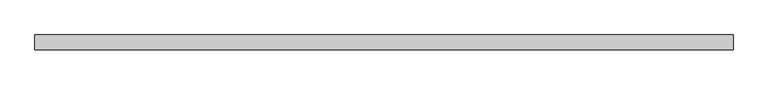
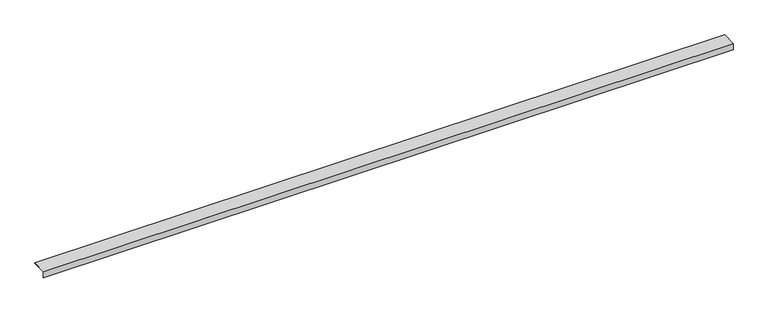
"""IFC4 building model written with IfcOpenShell, lengths in millimetres: proxy geometry, Generic Models 7:Generic Models 1:8:Generic Models 1:8 : Generic Models 7:Generic Models 1:337419:17 : Generic Models 7:Generic Models 1:8:Generic Models 1:8 : Generic Models 7:Generic Models 1:337419:315935."""

import ifcopenshell
import ifcopenshell.guid

model = None  # the IFC model being written
_history = None  # IfcOwnerHistory: only IFC2X3 demands one
_inside = {}  # id of a spatial element -> (the spatial element, [elements in it])
_under = {}  # id of a project, library or spatial element -> (it, [spatial elements below it])
_declared = {}  # id of a project -> (the project, [libraries it declares])
_typed = {}  # id of a type object -> (the type object, [elements of that type])
_made_of = {}  # id of a material, layer set ... -> (it, [elements and type objects made of it])


def new_model(schema):
    """Start an empty IFC model of exactly this schema.

    Asked for "IFC4X3", IfcOpenShell would pick the latest addendum, in which some entities
    have other attributes; the version numbers below select the first issue.
    IFC2X3 requires an IfcOwnerHistory on every rooted entity: one is made here for all.
    """
    global model, _history
    if schema == "IFC4X3":
        model = ifcopenshell.file(schema_version=(4, 3, 0, 0))
    else:
        model = ifcopenshell.file(schema=schema)
    _inside.clear()
    _under.clear()
    _declared.clear()
    _typed.clear()
    _made_of.clear()
    _history = None
    if model.schema == "IFC2X3":
        org = make("IfcOrganization", Name="unknown")
        user = make(
            "IfcPersonAndOrganization",
            ThePerson=make("IfcPerson", FamilyName="unknown"),
            TheOrganization=org,
        )
        app = make(
            "IfcApplication",
            ApplicationDeveloper=org,
            Version="unknown",
            ApplicationFullName="unknown",
            ApplicationIdentifier="unknown",
        )
        _history = make(
            "IfcOwnerHistory",
            OwningUser=user,
            OwningApplication=app,
            ChangeAction="ADDED",
            CreationDate=0,
        )
    return model


def make(cls, **values):
    """One entity of the class cls with the attributes given. An attribute that is None is left unset."""
    return model.create_entity(
        cls, **{name: value for name, value in values.items() if value is not None}
    )


def rooted(cls, **values):
    """An entity with a GlobalId (a new one), such as an element, a storey or a relation."""
    return make(cls, GlobalId=ifcopenshell.guid.new(), OwnerHistory=_history, **values)


def si_unit(unit_type, name, prefix=None):
    """IfcSIUnit, for example si_unit("LENGTHUNIT", "METRE", prefix="MILLI")."""
    return make("IfcSIUnit", UnitType=unit_type, Prefix=prefix, Name=name)


def assignment(units):
    """IfcUnitAssignment: the units of a project."""
    return None if units is None else make("IfcUnitAssignment", Units=units)


def point(xyz):
    """IfcCartesianPoint."""
    return None if xyz is None else make("IfcCartesianPoint", Coordinates=xyz)


def direction(xyz):
    """IfcDirection."""
    return None if xyz is None else make("IfcDirection", DirectionRatios=xyz)


def frame(location, z_axis=None, x_axis=None):
    """IfcAxis2Placement3D, a coordinate frame: its origin and axes. An axis left out is left unset."""
    return make(
        "IfcAxis2Placement3D",
        Location=point(location),
        Axis=direction(z_axis),
        RefDirection=direction(x_axis),
    )


def origin():
    """The frame at (0, 0, 0) with its axes left unset."""
    return frame((0.0, 0.0, 0.0))


def place(relative_to, where):
    """IfcLocalPlacement: puts the frame where relative to a parent placement (None: the world)."""
    return make(
        "IfcLocalPlacement", PlacementRelTo=relative_to, RelativePlacement=where
    )


def context(
    kind, dimensions, precision=None, world=None, true_north=None, identifier=None
):
    """IfcGeometricRepresentationContext, for example the 3D "Model" context."""
    return make(
        "IfcGeometricRepresentationContext",
        ContextIdentifier=identifier,
        ContextType=kind,
        CoordinateSpaceDimension=dimensions,
        Precision=precision,
        WorldCoordinateSystem=world,
        TrueNorth=true_north,
    )


def project(units=None, contexts=None):
    """IfcProject with its units and contexts."""
    return rooted(
        "IfcProject",
        Name="project",
        RepresentationContexts=contexts,
        UnitsInContext=assignment(units),
    )


def spatial(cls, under=None, at=None, **own):
    """A site, building, storey or space (cls), placed at a placement, below another one or the project."""
    s = rooted(cls, ObjectPlacement=at, **own)
    if under is not None:
        _under.setdefault(under.id(), (under, []))[1].append(s)
    return s


def polyline(points):
    """IfcPolyline through the points."""
    return make("IfcPolyline", Points=[point(p) for p in points])


def outline(outer, holes=None, kind="AREA"):
    """IfcArbitraryClosedProfileDef: a profile drawn as a closed curve; with holes, ...WithVoids."""
    if holes is None:
        return make("IfcArbitraryClosedProfileDef", ProfileType=kind, OuterCurve=outer)
    return make(
        "IfcArbitraryProfileDefWithVoids",
        ProfileType=kind,
        OuterCurve=outer,
        InnerCurves=holes,
    )


def extrude(swept, where, along, depth):
    """IfcExtrudedAreaSolid: the profile swept, set in the frame where, extruded along a direction by depth."""
    return make(
        "IfcExtrudedAreaSolid",
        SweptArea=swept,
        Position=where,
        ExtrudedDirection=direction(along),
        Depth=depth,
    )


def shape(context_of_items, identifier, shape_type, items):
    """IfcShapeRepresentation: the items that make up one representation, for example the "Body"."""
    return make(
        "IfcShapeRepresentation",
        ContextOfItems=context_of_items,
        RepresentationIdentifier=identifier,
        RepresentationType=shape_type,
        Items=items,
    )


def source(mapping_origin, context_of_items, identifier, shape_type, items):
    """IfcRepresentationMap: a shape defined once, which mapped items show again and again."""
    return make(
        "IfcRepresentationMap",
        MappingOrigin=mapping_origin,
        MappedRepresentation=shape(context_of_items, identifier, shape_type, items),
    )


def transform(
    local_origin,
    x_axis=None,
    y_axis=None,
    z_axis=None,
    scale=None,
    scale2=None,
    scale3=None,
    uniform=True,
):
    """IfcCartesianTransformationOperator3D, or its non-uniform kind. x_axis, y_axis, z_axis: its Axis1, 2, 3."""
    if uniform:
        return make(
            "IfcCartesianTransformationOperator3D",
            Axis1=direction(x_axis),
            Axis2=direction(y_axis),
            LocalOrigin=point(local_origin),
            Scale=scale,
            Axis3=direction(z_axis),
        )
    return make(
        "IfcCartesianTransformationOperator3DnonUniform",
        Axis1=direction(x_axis),
        Axis2=direction(y_axis),
        LocalOrigin=point(local_origin),
        Scale=scale,
        Axis3=direction(z_axis),
        Scale2=scale2,
        Scale3=scale3,
    )


def mapped(mapping_source, mapping_target):
    """IfcMappedItem: shows the shape of a source again, moved by a transform."""
    return make(
        "IfcMappedItem", MappingSource=mapping_source, MappingTarget=mapping_target
    )


def made_of(thing, what):
    """Note that an element or type object is made of a material, layer set ...; save() writes the relation."""
    if what is not None:
        _made_of.setdefault(what.id(), (what, []))[1].append(thing)
    return thing


def element(
    cls,
    number,
    at=None,
    inside=None,
    cuts=None,
    type_object=None,
    material=None,
    context=None,
    identifier="Body",
    shape_type=None,
    held_by="IfcProductDefinitionShape",
    body=None,
    shapes=None,
    **own,
):
    """One element of the class cls, such as IfcWall. Its Tag is "e" and its number.

    at: its placement. inside: the storey or other place that contains it. cuts: it is an
    opening in that element (IfcRelVoidsElement). A single representation is given by context,
    identifier, shape_type and body (its items); several are given by shapes. held_by: the class
    of the entity that holds the representations. save() writes the other relations.
    """
    e = rooted(cls, Tag="e%d" % number, ObjectPlacement=at, **own)
    if body is not None:
        shapes = [shape(context, identifier, shape_type, body)]
    if shapes is not None:
        e.Representation = make(held_by, Representations=shapes)
    if inside is not None:
        _inside.setdefault(inside.id(), (inside, []))[1].append(e)
    if cuts is not None:
        rooted(
            "IfcRelVoidsElement", RelatingBuildingElement=cuts, RelatedOpeningElement=e
        )
    if type_object is not None:
        _typed.setdefault(type_object.id(), (type_object, []))[1].append(e)
    return made_of(e, material)


def aggregate(whole, parts):
    """IfcRelAggregates: a whole, such as a stair, and the parts it consists of."""
    return rooted("IfcRelAggregates", RelatingObject=whole, RelatedObjects=parts)


def save(model, path):
    """Write the relations noted so far, then the file.

    IfcRelAggregates (storeys below a building ...), IfcRelContainedInSpatialStructure (elements
    in a storey), IfcRelDefinesByType, IfcRelAssociatesMaterial and IfcRelDeclares: one each for
    every whole, place, type object, material and project.
    """
    for whole, parts in _under.values():
        aggregate(whole, parts)
    for where, things in _inside.values():
        rooted(
            "IfcRelContainedInSpatialStructure",
            RelatedElements=things,
            RelatingStructure=where,
        )
    for kind, things in _typed.values():
        rooted("IfcRelDefinesByType", RelatedObjects=things, RelatingType=kind)
    for what, things in _made_of.values():
        rooted("IfcRelAssociatesMaterial", RelatedObjects=things, RelatingMaterial=what)
    for by, libraries in _declared.values():
        rooted("IfcRelDeclares", RelatingContext=by, RelatedDefinitions=libraries)
    model.write(path)


def generic_models_8358865d(model_context):
    return source(origin(), model_context, "Body", "SweptSolid", [
        extrude(outline(polyline([(-579120.6092291, 3671.5071615), (-579124.1195091, 3671.5071615), (-579124.1195091, 3715.9571615), (-579021.2760575, 3720.2423053), (-579021.1299226, 3716.7350684), (-579120.6092291, 3712.5900973), (-579120.6092291, 3671.5071615)])), frame((591306.0367239, 0.0, 0.0), z_axis=(1.0, 0.0, 0.0), x_axis=(0.0, 1.0, 0.0)), (0.0, 0.0, 1.0), 4876.8),
    ])


if __name__ == "__main__":
    model = new_model("IFC4")
    model_context = context("Model", 3, world=origin())
    ifc_project = project(units=[si_unit("LENGTHUNIT", "METRE", prefix="MILLI")], contexts=[model_context])
    site = spatial("IfcSite", under=ifc_project)
    building = spatial("IfcBuilding", under=site)
    placement = place(None, origin())
    generic_models_shape = generic_models_8358865d(model_context)
    element("IfcBuildingElementProxy", 1, Name="Generic Models 7:Generic Models 1:8:Generic Models 1:8 : Generic Models 7:Generic Models 1:337419:17 : Generic Models 7:Generic Models 1:8:Generic Models 1:8 : Generic Models 7:Generic Models 1:337419:315935", ObjectType="Generic Models 7:Generic Models 1:8:Generic Models 1:8 : Generic Models 7:Generic Models 1:337419:17 : Generic Models 7:Generic Models 1:8:Generic Models 1:8 : Generic Models 7:Generic Models 1:337419:315935", at=placement, inside=building, context=model_context, shape_type="MappedRepresentation", body=[
        mapped(generic_models_shape, transform((0.0, 0.0, 0.0), x_axis=(1.0, 0.0, 0.0), y_axis=(0.0, 1.0, 0.0), z_axis=(0.0, 0.0, 1.0))),
    ])
    save(model, "model.ifc")

# Revit data of these elements
# Type "Generic Models 7:Generic Models 1:8:Generic Models 1:8 : Generic Models 7:Generic Models 1:337419:17 : Generic Models 7:Generic Models 1:8:Generic Models 1:8 : Generic Models 7:Generic Models 1:337419:315935"
#   NameOverride = "Generic Models 7:Generic Models 1:8:Generic Models 1:8 : Generic Models 7:Generic Models 1:337419:315935"
#   ObjectTypeOverride = "Generic Models 1:8 : Generic Models 7:Generic Models 1:337419"
#   Reference = "Generic Models 1"
#   Tag = "315935"
# Element 1 (IfcBuildingElementProxy, "Generic Models 7:Generic Models 1:8:Generic Models 1:8 : Generic Models 7:Generic Models 1:337419:17 : Generic Models 7:Generic Models 1:8:Generic Models 1:8 : Generic Models 7:Generic Models 1:337419:315935")
#   Materials on its faces: "11 GA. ALUM. BRAKE METAL"
# Materials
#   "11 GA. ALUM. BRAKE METAL": class "Unassigned", colour RGB 210 209 208, transparency 0, Cost = 0
